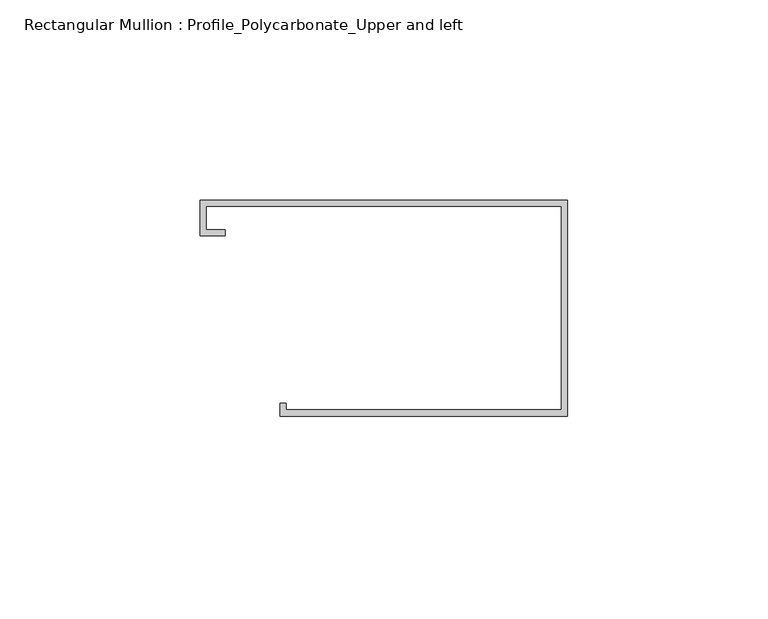
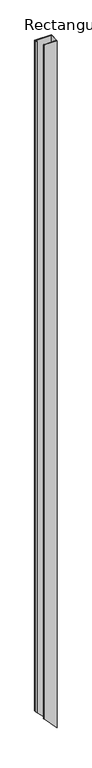
"""IFC4 building model written with IfcOpenShell, lengths in millimetres: member geometry, Rectangular Mullion : Profile_Polycarbonate_Upper and left."""

from ifc_helpers import new_model, si_unit, origin, place, context, project, spatial, faceted_brep, source, transform, mapped, element, save


def rectangular_mullion_profile_polycarbonate_upper_and_left_470a7b1e(model_context):
    return source(origin(), model_context, "Body", "Brep", [
        faceted_brep([(0.0, 28.984575, 0.0), (-91.9988, 28.984575, 0.0), (-91.9988, 19.992975, 0.0), (-85.6488, 19.992975, 0.0), (-85.6488, 21.580475, 0.0), (-90.4113, 21.580475, 0.0), (-90.4113, 27.397075, 0.0), (-1.5875, 27.397075, 0.0), (-1.5875, -23.428325, 0.0), (-70.3961, -23.428325, 0.0), (-70.3961, -21.840825, 0.0), (-71.9836, -21.840825, 0.0), (-71.9836, -25.015825, 0.0), (0.0, -25.015825, 0.0), (0.0, 28.984575, -3978.9266883), (-91.9988, 28.984575, -3883.0147795), (-91.9988, 19.992975, -3883.0147795), (-85.6488, 19.992975, -3889.6348726), (-85.6488, 21.580475, -3889.6348726), (-90.4113, 21.580475, -3884.6698028), (-90.4113, 27.397075, -3884.6698028), (-1.5875, 27.397075, -3977.271665), (-1.5875, -23.428325, -3977.271665), (-70.3961, -23.428325, -3905.5363363), (-70.3961, -21.840825, -3905.5363363), (-71.9836, -21.840825, -3903.881313), (-71.9836, -25.015825, -3903.881313), (0.0, -25.015825, -3978.9266883)], [[[0, 1, 2, 3, 4, 5, 6, 7, 8, 9, 10, 11, 12, 13]], [[1, 0, 14, 15]], [[2, 1, 15, 16]], [[3, 2, 16, 17]], [[4, 3, 17, 18]], [[5, 4, 18, 19]], [[6, 5, 19, 20]], [[7, 6, 20, 21]], [[8, 7, 21, 22]], [[9, 8, 22, 23]], [[10, 9, 23, 24]], [[11, 10, 24, 25]], [[12, 11, 25, 26]], [[13, 12, 26, 27]], [[0, 13, 27, 14]], [[14, 27, 26, 25, 24, 23, 22, 21, 20, 19, 18, 17, 16, 15]]]),
    ])


if __name__ == "__main__":
    model = new_model("IFC4")
    model_context = context("Model", 3, world=origin())
    ifc_project = project(units=[si_unit("LENGTHUNIT", "METRE", prefix="MILLI")], contexts=[model_context])
    site = spatial("IfcSite", under=ifc_project)
    building = spatial("IfcBuilding", under=site)
    placement = place(None, origin())
    rectangular_mullion_profile_polycarbonate_upper_and_left_shape = rectangular_mullion_profile_polycarbonate_upper_and_left_470a7b1e(model_context)
    element("IfcMember", 1, ObjectType="Rectangular Mullion : Profile_Polycarbonate_Upper and left", at=placement, inside=building, context=model_context, shape_type="MappedRepresentation", body=[
        mapped(rectangular_mullion_profile_polycarbonate_upper_and_left_shape, transform((0.0, 0.0, 0.0), x_axis=(1.0, 0.0, 0.0), y_axis=(0.0, 1.0, 0.0), z_axis=(0.0, 0.0, 1.0))),
    ])
    save(model, "model.ifc")

# Revit data of these elements
# Type "Rectangular Mullion : Profile_Polycarbonate_Upper and left"
#   built-in parameter 1007322 = 0.177167 (stored number, unit not read)
#   built-in parameter 1007321 = 0.00520833 (stored number, unit not read)
#   built-in parameter 1007320 = 0 (stored number, unit not read)
